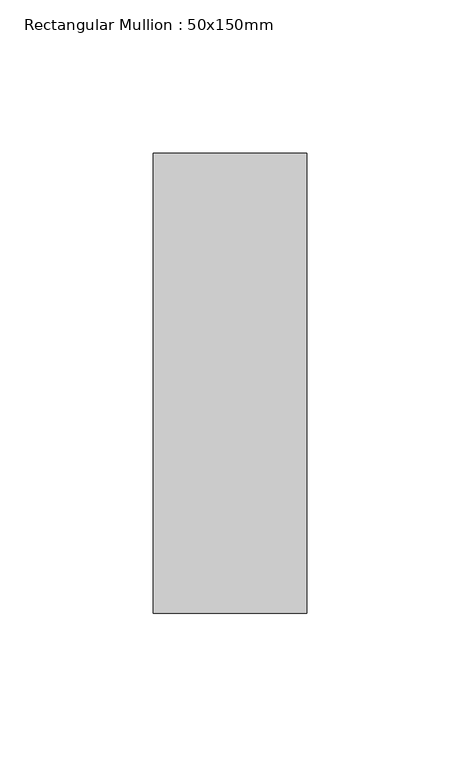
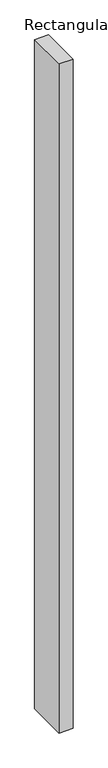
"""IFC4 building model written with IfcOpenShell, lengths in millimetres: member geometry, Rectangular Mullion : 50x150mm."""

from ifc_helpers import new_model, si_unit, frame, origin, place, context, project, spatial, polyline, outline, extrude, source, transform, mapped, element, save


def rectangular_mullion_50x150mm_4e17ee57(model_context):
    return source(origin(), model_context, "Body", "SweptSolid", [
        extrude(outline(polyline([(0.0, 75.0), (0.0, -75.0), (-50.0, -75.0), (-50.0, 75.0), (0.0, 75.0)])), frame((0.0, 0.0, -2522.0381538), z_axis=(0.0, 0.0, 1.0), x_axis=(1.0, 0.0, 0.0)), (0.0, 0.0, 1.0), 2522.0381538),
    ])


if __name__ == "__main__":
    model = new_model("IFC4")
    model_context = context("Model", 3, world=origin())
    ifc_project = project(units=[si_unit("LENGTHUNIT", "METRE", prefix="MILLI")], contexts=[model_context])
    site = spatial("IfcSite", under=ifc_project)
    building = spatial("IfcBuilding", under=site)
    placement = place(None, origin())
    rectangular_mullion_50x150mm_shape = rectangular_mullion_50x150mm_4e17ee57(model_context)
    element("IfcMember", 1, ObjectType="Rectangular Mullion : 50x150mm", at=placement, inside=building, context=model_context, shape_type="MappedRepresentation", body=[
        mapped(rectangular_mullion_50x150mm_shape, transform((0.0, 0.0, 0.0), x_axis=(1.0, 0.0, 0.0), y_axis=(0.0, 1.0, 0.0), z_axis=(0.0, 0.0, 1.0))),
    ])
    save(model, "model.ifc")

# Revit data of these elements
# Type "Rectangular Mullion : 50x150mm"
#   Keynote = "H11"
#   built-in parameter 1007304 = 0.492126 (stored number, unit not read)
#   built-in parameter 1007301 = 0.082021 (stored number, unit not read)
#   built-in parameter 1007300 = 0.082021 (stored number, unit not read)
# Element 1 (IfcMember, "Rectangular Mullion : 50x150mm")
#   Materials on its faces: "Aluminium"
# Materials
#   "Aluminium": class "Metal", colour RGB 247 247 247, transparency 0, Description = "Aluminium 6061", Cost = 0
